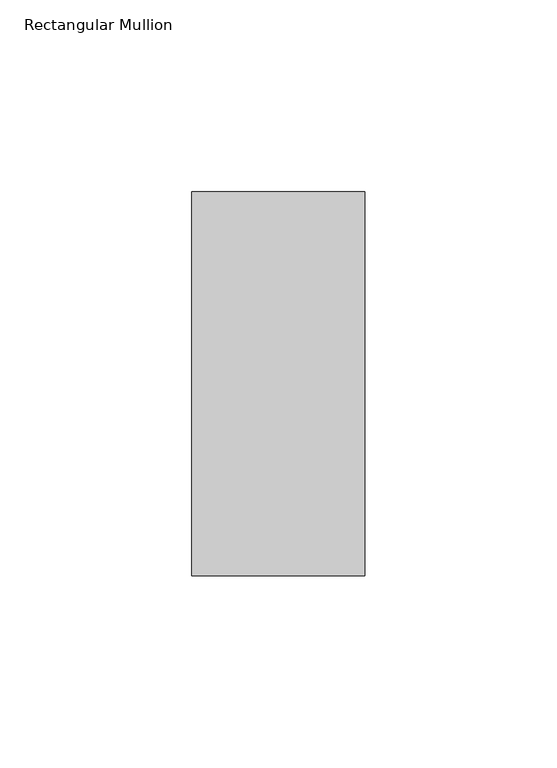
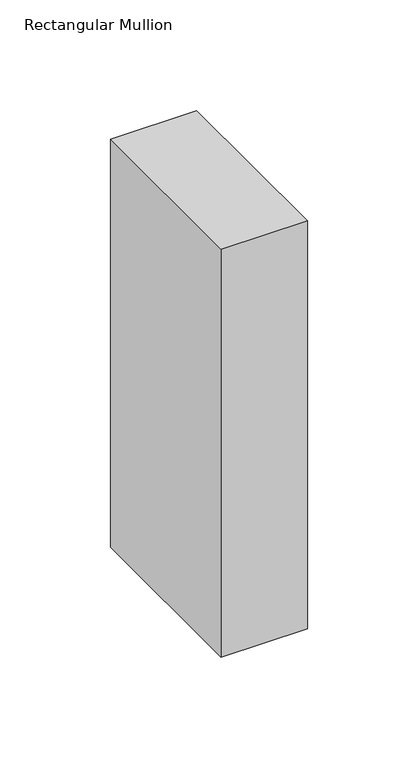
"""IFC4 building model written with IfcOpenShell, lengths in millimetres: member geometry, Rectangular Mullion : 알루미늄_Rectangular Cap_100 x 45."""

from ifc_helpers import new_model, si_unit, frame, origin, place, context, project, spatial, polyline, outline, extrude, source, transform, mapped, element, save


def rectangular_mullion_f3a363f7(model_context):
    return source(origin(), model_context, "Body", "SweptSolid", [
        extrude(outline(polyline([(0.0, 50.0), (0.0, -50.0), (-45.0, -50.0), (-45.0, 50.0), (0.0, 50.0)])), frame((0.0, 0.0, -225.0), z_axis=(0.0, 0.0, 1.0), x_axis=(1.0, 0.0, 0.0)), (0.0, 0.0, 1.0), 225.0),
    ])


if __name__ == "__main__":
    model = new_model("IFC4")
    model_context = context("Model", 3, world=origin())
    ifc_project = project(units=[si_unit("LENGTHUNIT", "METRE", prefix="MILLI")], contexts=[model_context])
    site = spatial("IfcSite", under=ifc_project)
    building = spatial("IfcBuilding", under=site)
    placement = place(None, origin())
    rectangular_mullion_shape = rectangular_mullion_f3a363f7(model_context)
    element("IfcMember", 1, ObjectType="Rectangular Mullion : 알루미늄_Rectangular Cap_100 x 45", at=placement, inside=building, context=model_context, shape_type="MappedRepresentation", body=[
        mapped(rectangular_mullion_shape, transform((0.0, 0.0, 0.0), x_axis=(1.0, 0.0, 0.0), y_axis=(0.0, 1.0, 0.0), z_axis=(0.0, 0.0, 1.0))),
    ])
    save(model, "model.ifc")

# Revit data of these elements
# Type "Rectangular Mullion : 알루미늄_Rectangular Cap_100 x 45"
#   built-in parameter 1007304 = 0.328084 (stored number, unit not read)
#   built-in parameter 1007301 = 0.0738189 (stored number, unit not read)
#   built-in parameter 1007300 = 0.0738189 (stored number, unit not read)
# Element 1 (IfcMember, "Rectangular Mullion : 알루미늄_Rectangular Cap_100 x 45")
#   Materials on its faces: "00_Metal_Stainless Steel"
# Materials
#   "00_Metal_Stainless Steel": class "Metal", colour RGB 148 148 148, transparency 0, Description = "Steel", Cost = 0
